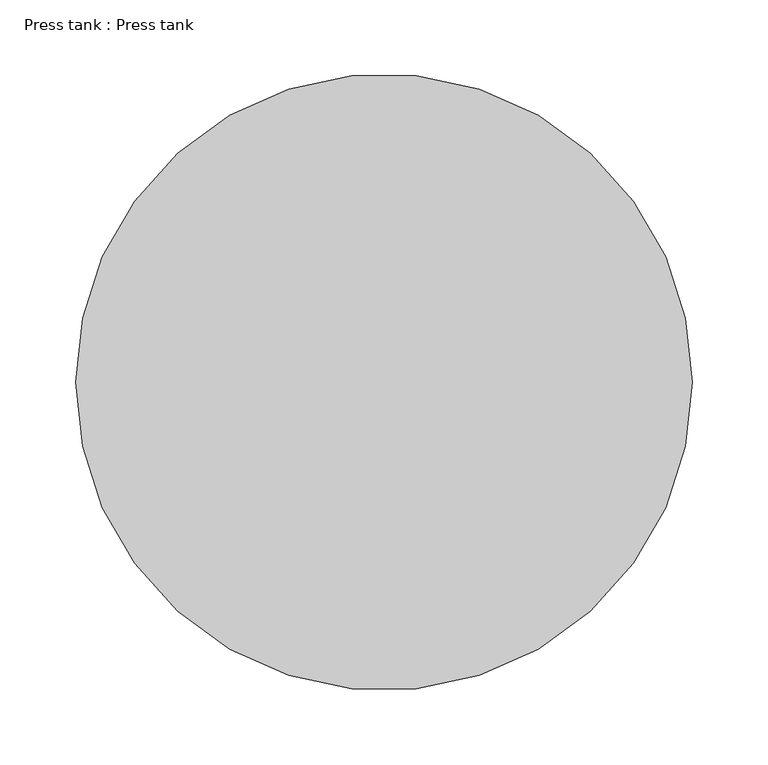
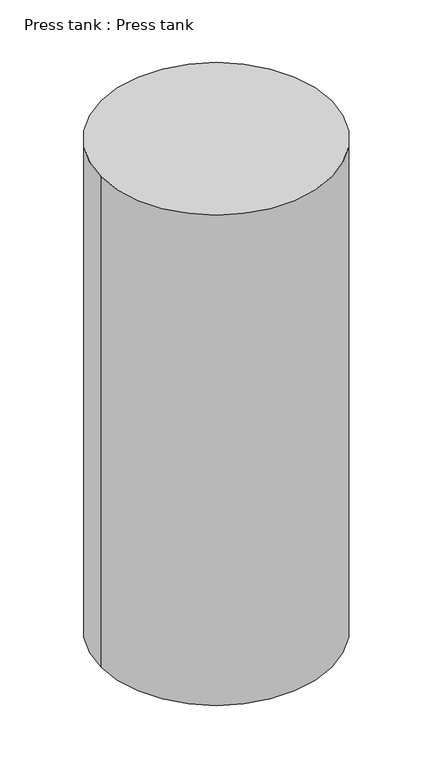
"""IFC4 building model written with IfcOpenShell, lengths in millimetres: proxy geometry, Press tank : Press tank."""

from ifc_helpers import new_model, si_unit, point, frame, frame_2d, origin, place, context, project, spatial, circle_curve, trimmed, segment, composite_curve, outline, extrude, source, transform, mapped, element, save


def press_tank_press_tank_b5f43448(model_context):
    return source(origin(), model_context, "Body", "SweptSolid", [
        extrude(outline(composite_curve([segment(trimmed(circle_curve(frame_2d((23819.6370052, 10524.1286841)), 203.2), [point((23616.4370052, 10524.1286841))], [point((24022.8370052, 10524.1286841))], False, "CARTESIAN"), True, "CONTINUOUS"), segment(trimmed(circle_curve(frame_2d((23819.6370052, 10524.1286841)), 203.2), [point((24022.8370052, 10524.1286841))], [point((23616.4370052, 10524.1286841))], False, "CARTESIAN"), True, "CONTINUOUS")], self_intersect=False)), frame((0.0, 0.0, 2832.1), z_axis=(0.0, 0.0, 1.0), x_axis=(1.0, 0.0, 0.0)), (0.0, 0.0, 1.0), 914.4),
    ])


if __name__ == "__main__":
    model = new_model("IFC4")
    model_context = context("Model", 3, world=origin())
    ifc_project = project(units=[si_unit("LENGTHUNIT", "METRE", prefix="MILLI")], contexts=[model_context])
    site = spatial("IfcSite", under=ifc_project)
    building = spatial("IfcBuilding", under=site)
    placement = place(None, origin())
    press_tank_press_tank_shape = press_tank_press_tank_b5f43448(model_context)
    element("IfcBuildingElementProxy", 1, Name="Press tank : Press tank", ObjectType="Press tank : Press tank", at=placement, inside=building, context=model_context, shape_type="MappedRepresentation", body=[
        mapped(press_tank_press_tank_shape, transform((0.0, 0.0, 0.0), x_axis=(1.0, 0.0, 0.0), y_axis=(0.0, 1.0, 0.0), z_axis=(0.0, 0.0, 1.0))),
    ])
    save(model, "model.ifc")
